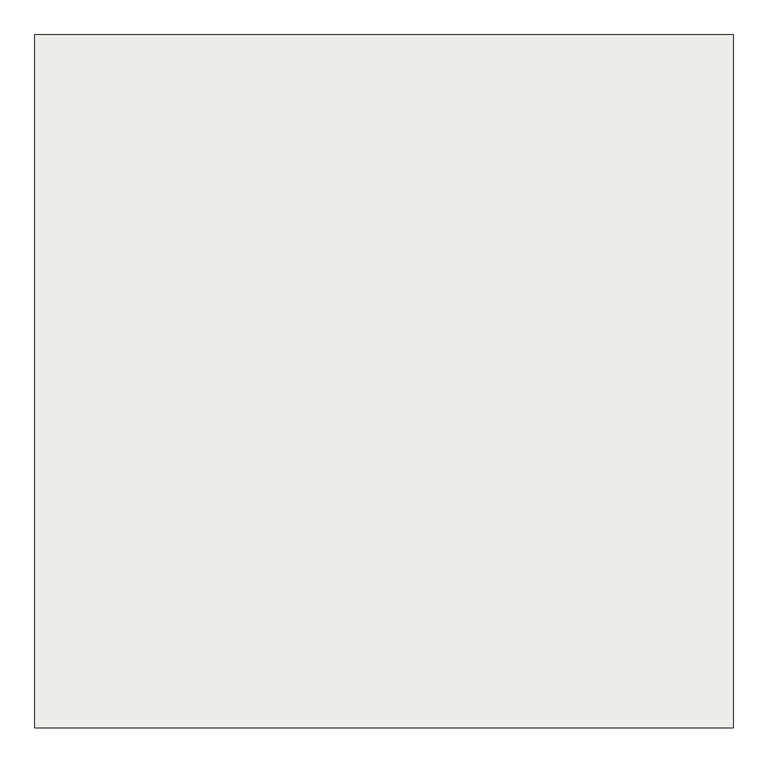
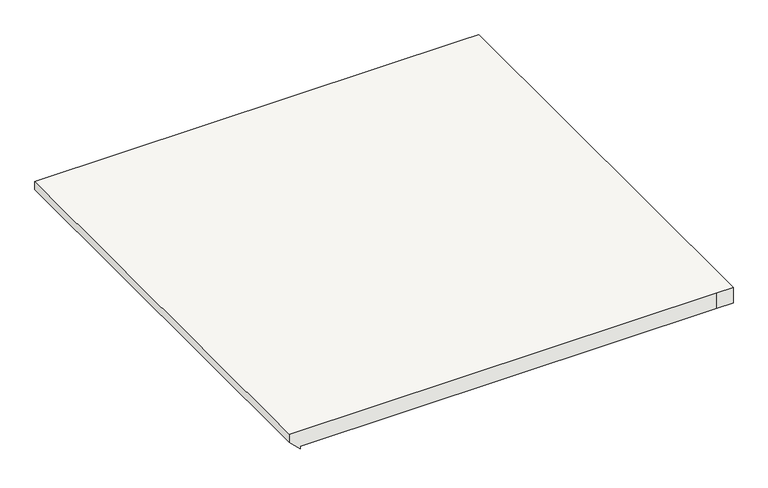
"""IFC4 building model written with IfcOpenShell, lengths in millimetres: slab geometry."""

from ifc_helpers import new_model, si_unit, origin, place, context, project, spatial, faceted_brep, source, transform, mapped, element, save


def slab_e4f51759(model_context):
    return source(origin(), model_context, "Body", "Brep", [
        faceted_brep([(-3903.6361778, 8211.7063821, 1392.7147059), (-3903.6361778, 8211.7063821, 1411.7647059), (-3903.6361778, 9211.7063821, 1411.7647059), (-3903.6361778, 9211.7063821, 1392.7147059), (-3878.2361778, 8211.7063821, 1367.3147059), (-3878.2361778, 9211.7063821, 1367.3147059), (-3878.2361778, 9211.7063821, 1373.7647059), (-3878.2361778, 8211.7063821, 1373.7647059), (-2934.2155657, 8211.7063821, 1411.7647059), (-2896.2155657, 8211.7063821, 1411.7647059), (-2896.2155657, 9211.7063821, 1411.7647059), (-2934.2155657, 9211.7063821, 1411.7647059), (-2934.2155657, 8211.7063821, 1373.7647059), (-2934.2155657, 9211.7063821, 1373.7647059), (-2896.2155657, 9211.7063821, 1373.7647059), (-2896.2155657, 8211.7063821, 1373.7647059)], [[[0, 1, 2, 3]], [[4, 0, 3, 5]], [[4, 5, 6, 7]], [[8, 9, 10, 11, 2, 1]], [[12, 7, 6, 13, 14, 15]], [[8, 1, 0, 4, 7, 12]], [[9, 8, 12, 15]], [[10, 9, 15, 14]], [[11, 10, 14, 13]], [[2, 11, 13, 6, 5, 3]]]),
    ])


if __name__ == "__main__":
    model = new_model("IFC4")
    model_context = context("Model", 3, world=origin())
    ifc_project = project(units=[si_unit("LENGTHUNIT", "METRE", prefix="MILLI")], contexts=[model_context])
    site = spatial("IfcSite", under=ifc_project)
    building = spatial("IfcBuilding", under=site)
    placement = place(None, origin())
    slab_shape = slab_e4f51759(model_context)
    element("IfcSlab", 1, at=placement, inside=building, context=model_context, shape_type="MappedRepresentation", body=[
        mapped(slab_shape, transform((0.0, 0.0, 0.0), x_axis=(1.0, 0.0, 0.0), y_axis=(0.0, 1.0, 0.0), z_axis=(0.0, 0.0, 1.0))),
    ])
    save(model, "model.ifc")

# Revit data of these elements
# Element 1 (IfcSlab)
#   Materials on its faces: "Concrete, Cast-in-Place gray"
# Materials
#   "Concrete, Cast-in-Place gray": class "Concrete", colour RGB 192 192 192, transparency 0, Description = "Cast-in-place concrete", Cost = 0
